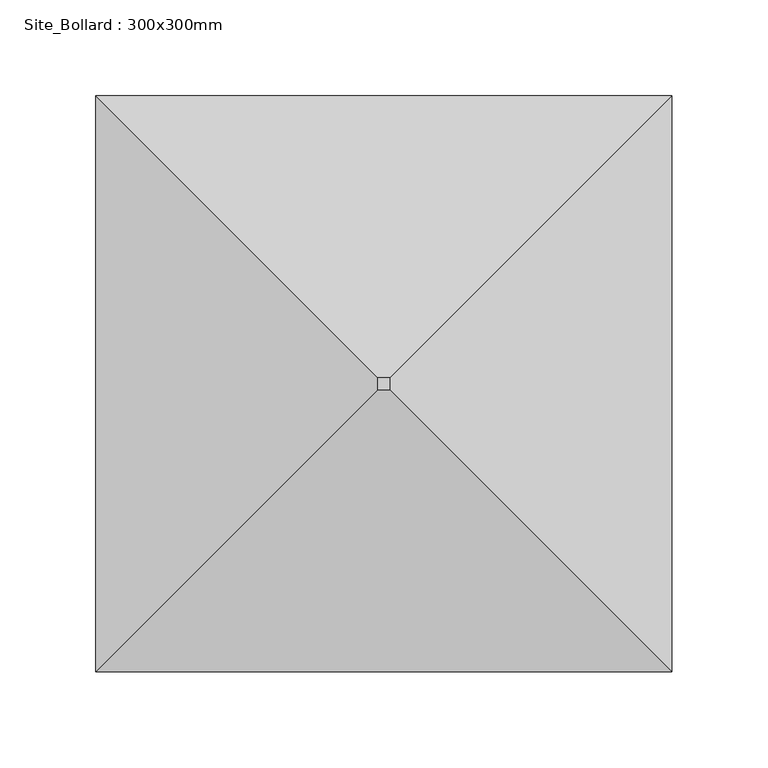
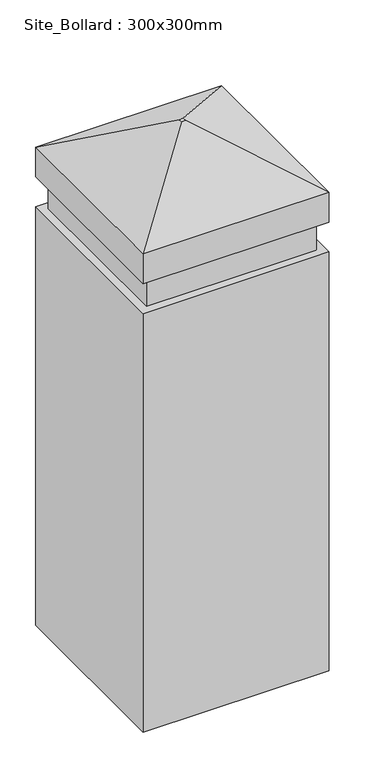
"""IFC4 building model written with IfcOpenShell, lengths in millimetres: geographic element geometry, Site_Bollard : 300x300mm."""

from ifc_helpers import new_model, si_unit, frame, origin, origin_with_axes, place, context, project, spatial, polyline, outline, extrude, faceted_brep, source, transform, mapped, element, save


def site_bollard_300x300mm_9e5afc0f(model_context):
    return source(origin(), model_context, "Body", "SolidModel", [
        faceted_brep([(5.575, 5.575, 900.0), (-0.775, 5.575, 900.0), (-0.775, -0.775, 900.0), (5.575, -0.775, 900.0), (152.4, 152.4, 815.18125), (152.4, -147.6, 815.18125), (-147.6, -147.6, 815.18125), (-147.6, 152.4, 815.18125)], [[[0, 1, 2, 3]], [[4, 5, 6, 7]], [[4, 7, 1, 0]], [[7, 6, 2, 1]], [[6, 5, 3, 2]], [[5, 4, 0, 3]]]),
        extrude(outline(polyline([(152.4, 152.4), (152.4, -147.6), (-147.6, -147.6), (-147.6, 152.4), (152.4, 152.4)])), frame((0.0, 0.0, 764.38125), z_axis=(0.0, 0.0, 1.0), x_axis=(1.0, 0.0, 0.0)), (0.0, 0.0, 1.0), 50.8),
        extrude(outline(polyline([(139.7, 139.7), (139.7, -134.9), (-134.9, -134.9), (-134.9, 139.7), (139.7, 139.7)])), frame((0.0, 0.0, 713.58125), z_axis=(0.0, 0.0, 1.0), x_axis=(1.0, 0.0, 0.0)), (0.0, 0.0, 1.0), 50.8),
        extrude(outline(polyline([(152.4, 152.4), (152.4, -147.6), (-147.6, -147.6), (-147.6, 152.4), (152.4, 152.4)])), origin_with_axes(), (0.0, 0.0, 1.0), 713.58125),
    ])


if __name__ == "__main__":
    model = new_model("IFC4")
    model_context = context("Model", 3, world=origin())
    ifc_project = project(units=[si_unit("LENGTHUNIT", "METRE", prefix="MILLI")], contexts=[model_context])
    site = spatial("IfcSite", under=ifc_project)
    building = spatial("IfcBuilding", under=site)
    placement = place(None, origin())
    site_bollard_300x300mm_shape = site_bollard_300x300mm_9e5afc0f(model_context)
    element("IfcGeographicElement", 1, ObjectType="Site_Bollard : 300x300mm", at=placement, inside=building, context=model_context, shape_type="MappedRepresentation", body=[
        mapped(site_bollard_300x300mm_shape, transform((0.0, 0.0, 0.0), x_axis=(1.0, 0.0, 0.0), y_axis=(0.0, 1.0, 0.0), z_axis=(0.0, 0.0, 1.0))),
    ])
    save(model, "model.ifc")

# Revit data of these elements
# Type "Site_Bollard : 300x300mm"
#   Material = Concrete - Precast Concrete
# Element 1 (IfcGeographicElement, "Site_Bollard : 300x300mm")
#   Materials on its faces: "Concrete - Precast Concrete"
# Materials
#   "Concrete - Precast Concrete": class "Concrete", colour RGB 198 187 187, transparency 0
